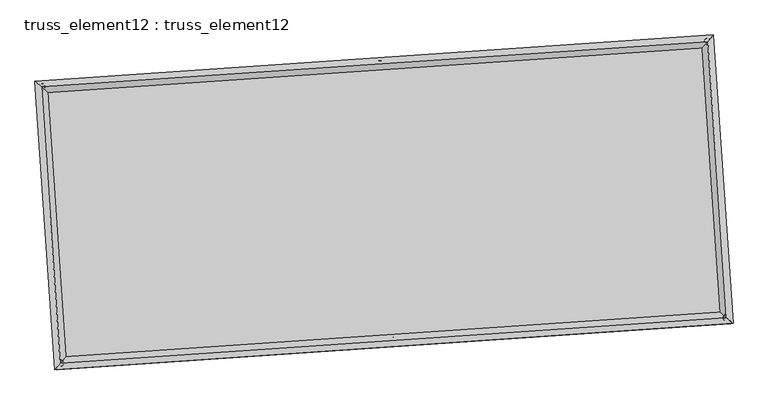
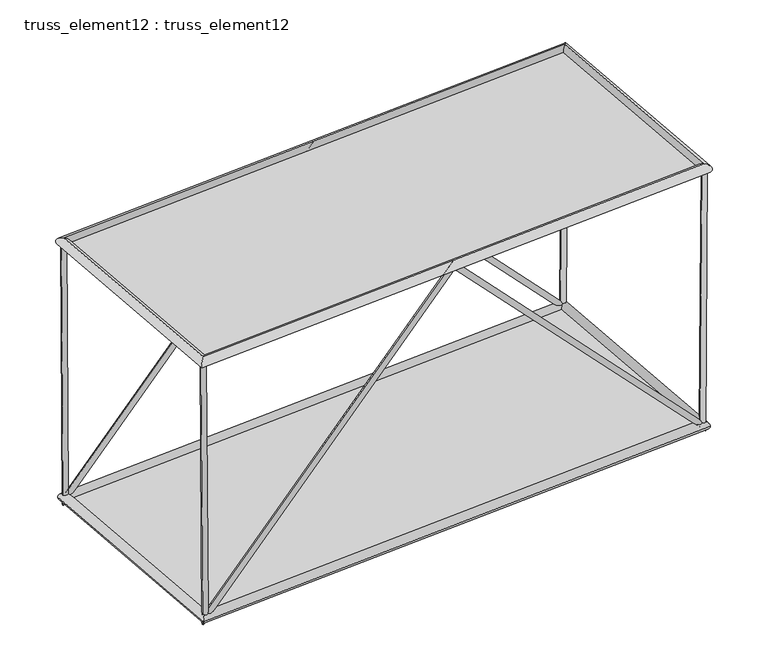
"""IFC4 building model written with IfcOpenShell, lengths in millimetres: plate geometry, truss_element12 : truss_element12."""

import ifcopenshell
import ifcopenshell.guid

model = None  # the IFC model being written
_history = None  # IfcOwnerHistory: only IFC2X3 demands one
_inside = {}  # id of a spatial element -> (the spatial element, [elements in it])
_under = {}  # id of a project, library or spatial element -> (it, [spatial elements below it])
_declared = {}  # id of a project -> (the project, [libraries it declares])
_typed = {}  # id of a type object -> (the type object, [elements of that type])
_made_of = {}  # id of a material, layer set ... -> (it, [elements and type objects made of it])


def new_model(schema):
    """Start an empty IFC model of exactly this schema.

    Asked for "IFC4X3", IfcOpenShell would pick the latest addendum, in which some entities
    have other attributes; the version numbers below select the first issue.
    IFC2X3 requires an IfcOwnerHistory on every rooted entity: one is made here for all.
    """
    global model, _history
    if schema == "IFC4X3":
        model = ifcopenshell.file(schema_version=(4, 3, 0, 0))
    else:
        model = ifcopenshell.file(schema=schema)
    _inside.clear()
    _under.clear()
    _declared.clear()
    _typed.clear()
    _made_of.clear()
    _history = None
    if model.schema == "IFC2X3":
        org = make("IfcOrganization", Name="unknown")
        user = make(
            "IfcPersonAndOrganization",
            ThePerson=make("IfcPerson", FamilyName="unknown"),
            TheOrganization=org,
        )
        app = make(
            "IfcApplication",
            ApplicationDeveloper=org,
            Version="unknown",
            ApplicationFullName="unknown",
            ApplicationIdentifier="unknown",
        )
        _history = make(
            "IfcOwnerHistory",
            OwningUser=user,
            OwningApplication=app,
            ChangeAction="ADDED",
            CreationDate=0,
        )
    return model


def make(cls, **values):
    """One entity of the class cls with the attributes given. An attribute that is None is left unset."""
    return model.create_entity(
        cls, **{name: value for name, value in values.items() if value is not None}
    )


def rooted(cls, **values):
    """An entity with a GlobalId (a new one), such as an element, a storey or a relation."""
    return make(cls, GlobalId=ifcopenshell.guid.new(), OwnerHistory=_history, **values)


def si_unit(unit_type, name, prefix=None):
    """IfcSIUnit, for example si_unit("LENGTHUNIT", "METRE", prefix="MILLI")."""
    return make("IfcSIUnit", UnitType=unit_type, Prefix=prefix, Name=name)


def assignment(units):
    """IfcUnitAssignment: the units of a project."""
    return None if units is None else make("IfcUnitAssignment", Units=units)


def point(xyz):
    """IfcCartesianPoint."""
    return None if xyz is None else make("IfcCartesianPoint", Coordinates=xyz)


def direction(xyz):
    """IfcDirection."""
    return None if xyz is None else make("IfcDirection", DirectionRatios=xyz)


def frame(location, z_axis=None, x_axis=None):
    """IfcAxis2Placement3D, a coordinate frame: its origin and axes. An axis left out is left unset."""
    return make(
        "IfcAxis2Placement3D",
        Location=point(location),
        Axis=direction(z_axis),
        RefDirection=direction(x_axis),
    )


def origin():
    """The frame at (0, 0, 0) with its axes left unset."""
    return frame((0.0, 0.0, 0.0))


def origin_with_axes():
    """The frame at (0, 0, 0) with the z axis (0, 0, 1) and the x axis (1, 0, 0) written out."""
    return frame((0.0, 0.0, 0.0), z_axis=(0.0, 0.0, 1.0), x_axis=(1.0, 0.0, 0.0))


def place(relative_to, where):
    """IfcLocalPlacement: puts the frame where relative to a parent placement (None: the world)."""
    return make(
        "IfcLocalPlacement", PlacementRelTo=relative_to, RelativePlacement=where
    )


def context(
    kind, dimensions, precision=None, world=None, true_north=None, identifier=None
):
    """IfcGeometricRepresentationContext, for example the 3D "Model" context."""
    return make(
        "IfcGeometricRepresentationContext",
        ContextIdentifier=identifier,
        ContextType=kind,
        CoordinateSpaceDimension=dimensions,
        Precision=precision,
        WorldCoordinateSystem=world,
        TrueNorth=true_north,
    )


def project(units=None, contexts=None):
    """IfcProject with its units and contexts."""
    return rooted(
        "IfcProject",
        Name="project",
        RepresentationContexts=contexts,
        UnitsInContext=assignment(units),
    )


def spatial(cls, under=None, at=None, **own):
    """A site, building, storey or space (cls), placed at a placement, below another one or the project."""
    s = rooted(cls, ObjectPlacement=at, **own)
    if under is not None:
        _under.setdefault(under.id(), (under, []))[1].append(s)
    return s


def polyline(points):
    """IfcPolyline through the points."""
    return make("IfcPolyline", Points=[point(p) for p in points])


def circle_curve(where, radius):
    """IfcCircle in the frame where."""
    return make("IfcCircle", Position=where, Radius=radius)


def ellipse_curve(where, semi_axis1, semi_axis2):
    """IfcEllipse in the frame where."""
    return make(
        "IfcEllipse", Position=where, SemiAxis1=semi_axis1, SemiAxis2=semi_axis2
    )


def outline(outer, holes=None, kind="AREA"):
    """IfcArbitraryClosedProfileDef: a profile drawn as a closed curve; with holes, ...WithVoids."""
    if holes is None:
        return make("IfcArbitraryClosedProfileDef", ProfileType=kind, OuterCurve=outer)
    return make(
        "IfcArbitraryProfileDefWithVoids",
        ProfileType=kind,
        OuterCurve=outer,
        InnerCurves=holes,
    )


def extrude(swept, where, along, depth):
    """IfcExtrudedAreaSolid: the profile swept, set in the frame where, extruded along a direction by depth."""
    return make(
        "IfcExtrudedAreaSolid",
        SweptArea=swept,
        Position=where,
        ExtrudedDirection=direction(along),
        Depth=depth,
    )


def shape(context_of_items, identifier, shape_type, items):
    """IfcShapeRepresentation: the items that make up one representation, for example the "Body"."""
    return make(
        "IfcShapeRepresentation",
        ContextOfItems=context_of_items,
        RepresentationIdentifier=identifier,
        RepresentationType=shape_type,
        Items=items,
    )


def source(mapping_origin, context_of_items, identifier, shape_type, items):
    """IfcRepresentationMap: a shape defined once, which mapped items show again and again."""
    return make(
        "IfcRepresentationMap",
        MappingOrigin=mapping_origin,
        MappedRepresentation=shape(context_of_items, identifier, shape_type, items),
    )


def transform(
    local_origin,
    x_axis=None,
    y_axis=None,
    z_axis=None,
    scale=None,
    scale2=None,
    scale3=None,
    uniform=True,
):
    """IfcCartesianTransformationOperator3D, or its non-uniform kind. x_axis, y_axis, z_axis: its Axis1, 2, 3."""
    if uniform:
        return make(
            "IfcCartesianTransformationOperator3D",
            Axis1=direction(x_axis),
            Axis2=direction(y_axis),
            LocalOrigin=point(local_origin),
            Scale=scale,
            Axis3=direction(z_axis),
        )
    return make(
        "IfcCartesianTransformationOperator3DnonUniform",
        Axis1=direction(x_axis),
        Axis2=direction(y_axis),
        LocalOrigin=point(local_origin),
        Scale=scale,
        Axis3=direction(z_axis),
        Scale2=scale2,
        Scale3=scale3,
    )


def mapped(mapping_source, mapping_target):
    """IfcMappedItem: shows the shape of a source again, moved by a transform."""
    return make(
        "IfcMappedItem", MappingSource=mapping_source, MappingTarget=mapping_target
    )


def made_of(thing, what):
    """Note that an element or type object is made of a material, layer set ...; save() writes the relation."""
    if what is not None:
        _made_of.setdefault(what.id(), (what, []))[1].append(thing)
    return thing


def element(
    cls,
    number,
    at=None,
    inside=None,
    cuts=None,
    type_object=None,
    material=None,
    context=None,
    identifier="Body",
    shape_type=None,
    held_by="IfcProductDefinitionShape",
    body=None,
    shapes=None,
    **own,
):
    """One element of the class cls, such as IfcWall. Its Tag is "e" and its number.

    at: its placement. inside: the storey or other place that contains it. cuts: it is an
    opening in that element (IfcRelVoidsElement). A single representation is given by context,
    identifier, shape_type and body (its items); several are given by shapes. held_by: the class
    of the entity that holds the representations. save() writes the other relations.
    """
    e = rooted(cls, Tag="e%d" % number, ObjectPlacement=at, **own)
    if body is not None:
        shapes = [shape(context, identifier, shape_type, body)]
    if shapes is not None:
        e.Representation = make(held_by, Representations=shapes)
    if inside is not None:
        _inside.setdefault(inside.id(), (inside, []))[1].append(e)
    if cuts is not None:
        rooted(
            "IfcRelVoidsElement", RelatingBuildingElement=cuts, RelatedOpeningElement=e
        )
    if type_object is not None:
        _typed.setdefault(type_object.id(), (type_object, []))[1].append(e)
    return made_of(e, material)


def aggregate(whole, parts):
    """IfcRelAggregates: a whole, such as a stair, and the parts it consists of."""
    return rooted("IfcRelAggregates", RelatingObject=whole, RelatedObjects=parts)


def save(model, path):
    """Write the relations noted so far, then the file.

    IfcRelAggregates (storeys below a building ...), IfcRelContainedInSpatialStructure (elements
    in a storey), IfcRelDefinesByType, IfcRelAssociatesMaterial and IfcRelDeclares: one each for
    every whole, place, type object, material and project.
    """
    for whole, parts in _under.values():
        aggregate(whole, parts)
    for where, things in _inside.values():
        rooted(
            "IfcRelContainedInSpatialStructure",
            RelatedElements=things,
            RelatingStructure=where,
        )
    for kind, things in _typed.values():
        rooted("IfcRelDefinesByType", RelatedObjects=things, RelatingType=kind)
    for what, things in _made_of.values():
        rooted("IfcRelAssociatesMaterial", RelatedObjects=things, RelatingMaterial=what)
    for by, libraries in _declared.values():
        rooted("IfcRelDeclares", RelatingContext=by, RelatedDefinitions=libraries)
    model.write(path)


def plane_surface(at):
    """IfcPlane: the flat surface through the origin of the frame at, square to its z axis."""
    return make("IfcPlane", Position=at)


def cylinder_surface(at, radius):
    """IfcCylindricalSurface: all points at the distance radius from the z axis of the frame at."""
    return make("IfcCylindricalSurface", Position=at, Radius=radius)


def advanced_brep(points, edges, surfaces, faces):
    """IfcAdvancedBrep: a solid bounded by faces that lie on surfaces and meet in shared edges.

    An edge is (start, end): straight between two places in points (the first is 0);
    or (start, end, curve); or (start, end, curve, False) where it runs against its curve.
    A face is (place in surfaces, loops), or (place, loops, False) where it looks against
    its surface's normal. A loop lists edges by number (the first is 1), with a minus sign
    where the edge is run from its end to its start. The first loop is the outer one.
    """
    corners = [point(p) for p in points]
    vertices = [make("IfcVertexPoint", VertexGeometry=c) for c in corners]
    made = []
    for start, end, *more in edges:
        made.append(
            make(
                "IfcEdgeCurve",
                EdgeStart=vertices[start],
                EdgeEnd=vertices[end],
                EdgeGeometry=more[0] if more else make("IfcPolyline", Points=[corners[start], corners[end]]),
                SameSense=more[1] if len(more) > 1 else True,
            )
        )
    hull = []
    for where, loops, *sense in faces:
        bounds = []
        for j, loop in enumerate(loops):
            ring = [make("IfcOrientedEdge", EdgeElement=made[abs(k) - 1], Orientation=k > 0) for k in loop]
            bounds.append(
                make(
                    "IfcFaceOuterBound" if j == 0 else "IfcFaceBound",
                    Bound=make("IfcEdgeLoop", EdgeList=ring),
                    Orientation=True,
                )
            )
        hull.append(make("IfcAdvancedFace", Bounds=bounds, FaceSurface=surfaces[where], SameSense=sense[0] if sense else True))
    return make("IfcAdvancedBrep", Outer=make("IfcClosedShell", CfsFaces=hull))


def truss_element12_truss_element12_8e9da1f8(model_context):
    return source(origin(), model_context, "Body", "SolidModel", [
        advanced_brep(
        [(-3698.7518615, 2273.9185866, 5000.223301), (-3797.8529392, 2260.5574847, 4999.5470243), (-3665.7745625, 2276.1671833, 123.3293266), (-3763.2123204, 2262.9194968, -123.3293266), (1063.9844604, 2598.6714715, 5072.0064402), (1064.4287053, 2592.0979868, 4927.7602832), (5793.2263236, 2921.1404966, 123.3255902), (5891.5346534, 2921.2399919, -123.3255902), (5826.7168605, 2923.424089, 5000.224961), (5926.7142716, 2923.6387563, 4999.5381605)],
        [
            (0, 1, circle_curve(frame((-3748.3024003, 2267.2380357, 4999.8851627), z_axis=(-0.0067617917796413095, -0.00046106087747684727, 0.9999770325336459), x_axis=(-0.13361106793445865, 0.9910337446995272, -0.0004465335886331621)), 50.0)),
            (1, 0, circle_curve(frame((-3748.3024003, 2267.2380357, 4999.8851627), z_axis=(-0.0067617917796413095, -0.00046106087747684727, 0.9999770325336459), x_axis=(-0.13361106793445865, 0.9910337446995272, -0.0004465335886331621)), 50.0)),
            (0, 2),
            (2, 3, ellipse_curve(frame((-3714.4934414, 2269.54334, 0.0), z_axis=(-0.9270371329382548, -0.06321113809700207, 0.3696031739231987), x_axis=(0.3687469497597502, 0.025143452765731104, 0.9291896974385251)), 133.0168379, 50.0)),
            (3, 1),
            (3, 2, ellipse_curve(frame((-3714.4934414, 2269.54334, 0.0), z_axis=(-0.9270371329382548, -0.06321113809700207, 0.3696031739231987), x_axis=(0.3687469497597502, 0.025143452765731104, 0.9291896974385251)), 133.0168379, 50.0)),
            (2, 4),
            (4, 5, ellipse_curve(frame((1064.2065829, 2595.3847292, 4999.8833617), z_axis=(-0.9976833956976204, -0.06802823820297674, 2.7500260085138387e-05), x_axis=(-2.74365528747556e-05, -1.8707942443931063e-06, -0.9999999996218679)), 72.2801261, 50.0)),
            (5, 3),
            (5, 4, ellipse_curve(frame((1064.2065829, 2595.3847292, 4999.8833617), z_axis=(-0.9976833956976204, -0.06802823820297674, 2.7500260085138387e-05), x_axis=(-2.74365528747556e-05, -1.8707942443931063e-06, -0.9999999996218679)), 72.2801261, 50.0)),
            (4, 6),
            (6, 7, ellipse_curve(frame((5842.3804885, 2921.1902443, 0.0), z_axis=(-0.9270667165570741, -0.0632131552915117, -0.3695286187160294), x_axis=(-0.3686725672674666, -0.0251383809063366, 0.9292193497500056)), 133.0085635, 50.0)),
            (7, 5),
            (7, 6, ellipse_curve(frame((5842.3804885, 2921.1902443, 0.0), z_axis=(-0.9270667165570741, -0.0632131552915117, -0.3695286187160294), x_axis=(-0.3686725672674666, -0.0251383809063366, 0.9292193497500056)), 133.0085635, 50.0)),
            (8, 9, circle_curve(frame((5876.715566, 2923.5314227, 4999.8815607), z_axis=(0.0068670155092968675, 0.0004682356836093084, 0.9999763121461127), x_axis=(-0.00214983747870396, 0.9999975862733836, -0.0004534823281307776)), 50.0)),
            (9, 8, circle_curve(frame((5876.715566, 2923.5314227, 4999.8815607), z_axis=(0.0068670155092968675, 0.0004682356836093084, 0.9999763121461127), x_axis=(-0.00214983747870396, 0.9999975862733836, -0.0004534823281307776)), 50.0)),
            (6, 8),
            (9, 7),
        ],
        [
            plane_surface(frame((-3748.3024003, 2317.2380303, 4999.9082162), z_axis=(-0.006761791779640632, -0.0004610608774721699, 0.9999770325336457), x_axis=(0.9999771388246477, -3.1176689248013658e-06, 0.006761791060906577))),
            cylinder_surface(frame((-3748.3024003, 2267.2380357, 4999.8851627), z_axis=(-0.006761791779641308, -0.00046106087747684716, 0.9999770325336457), x_axis=(-0.13361106793445865, 0.9910337446995272, -0.0004465335886331621)), 50.0),
            cylinder_surface(frame((-3714.4934414, 2269.54334, 0.0), z_axis=(-0.6901703766804573, -0.0470600944026198, -0.7221150868577476), x_axis=(-0.020414252830953418, 0.9987522052200565, -0.045577306298510874)), 50.0),
            cylinder_surface(frame((1064.2065829, 2595.3847292, 4999.8833617), z_axis=(-0.6901307509390454, -0.04705739247394453, 0.7221531336370857), x_axis=(-0.11534910612614199, 0.9922789584550205, -0.045574689503274965)), 50.0),
            plane_surface(frame((5876.715566, 2873.5314282, 4999.9049731), z_axis=(0.006867015509297537, 0.00046823568361033024, 0.9999763121461126), x_axis=(0.9999764217710311, -3.215457516247967e-06, -0.006867014756483772))),
            cylinder_surface(frame((5842.3804885, 2921.1902443, 0.0), z_axis=(-0.0068670155092968675, -0.0004682356836093084, -0.9999763121461127), x_axis=(-0.00214983747870396, 0.9999975862733836, -0.0004534823281307776)), 50.0),
        ],
        [
            (0, [[1, 2]]),
            (1, [[-1, 3, 4, 5]]),
            (1, [[-2, -5, 6, -3]]),
            (2, [[-4, 7, 8, 9]]),
            (2, [[-6, -9, 10, -7]]),
            (3, [[-8, 11, 12, 13]]),
            (3, [[-10, -13, 14, -11]]),
            (4, [[15, 16]]),
            (5, [[-12, 17, -16, 18]]),
            (5, [[-14, -18, -15, -17]]),
        ],
    ),
        advanced_brep(
        [(-3426.6389085, -1716.8149977, 5000.223301), (-3525.7399863, -1730.1760996, 4999.5470243), (-3393.6616095, -1714.566401, 123.3293266), (-3491.0993675, -1727.8140875, -123.3293266), (1336.0974133, -1392.0621128, 5072.0064402), (1336.5416582, -1398.6355975, 4927.7602832), (6065.3392765, -1069.5930877, 123.3255902), (6163.6476063, -1069.4935924, -123.3255902), (6098.8298134, -1067.3094953, 5000.224961), (6198.8272245, -1067.094828, 4999.5381605)],
        [
            (0, 1, circle_curve(frame((-3476.1894474, -1723.4955486, 4999.8851627), z_axis=(-0.006761791779640981, -0.00046106087747676796, 0.9999770325336458), x_axis=(-0.13361106793445865, 0.9910337446995272, -0.0004465335886331968)), 50.0)),
            (1, 0, circle_curve(frame((-3476.1894474, -1723.4955486, 4999.8851627), z_axis=(-0.006761791779640981, -0.00046106087747676796, 0.9999770325336458), x_axis=(-0.13361106793445865, 0.9910337446995272, -0.0004465335886331968)), 50.0)),
            (0, 2),
            (2, 3, ellipse_curve(frame((-3442.3804885, -1721.1902443, 0.0), z_axis=(-0.9270371329382548, -0.06321113809700199, 0.3696031739231986), x_axis=(0.3687469497597501, 0.025143452765731125, 0.9291896974385251)), 133.0168379, 50.0)),
            (3, 1),
            (3, 2, ellipse_curve(frame((-3442.3804885, -1721.1902443, 0.0), z_axis=(-0.9270371329382548, -0.06321113809700199, 0.3696031739231986), x_axis=(0.3687469497597501, 0.025143452765731125, 0.9291896974385251)), 133.0168379, 50.0)),
            (2, 4),
            (4, 5, ellipse_curve(frame((1336.3195358, -1395.3488551, 4999.8833617), z_axis=(-0.9976833956976204, -0.0680282382029767, 2.7500260084977895e-05), x_axis=(-2.7436552874601853e-05, -1.8707942444027149e-06, -0.9999999996218678)), 72.2801261, 50.0)),
            (5, 3),
            (5, 4, ellipse_curve(frame((1336.3195358, -1395.3488551, 4999.8833617), z_axis=(-0.9976833956976204, -0.0680282382029767, 2.7500260084977895e-05), x_axis=(-2.7436552874601853e-05, -1.8707942444027149e-06, -0.9999999996218678)), 72.2801261, 50.0)),
            (4, 6),
            (6, 7, ellipse_curve(frame((6114.4934414, -1069.54334, 0.0), z_axis=(-0.9270667165570744, -0.06321315529151138, -0.3695286187160292), x_axis=(-0.36867256726746617, -0.025138380906336657, 0.9292193497500058)), 133.0085635, 50.0)),
            (7, 5),
            (7, 6, ellipse_curve(frame((6114.4934414, -1069.54334, 0.0), z_axis=(-0.9270667165570744, -0.06321315529151138, -0.3695286187160292), x_axis=(-0.36867256726746617, -0.025138380906336657, 0.9292193497500058)), 133.0085635, 50.0)),
            (8, 9, circle_curve(frame((6148.828519, -1067.2021616, 4999.8815607), z_axis=(0.0068670155092972595, 0.00046823568360912634, 0.9999763121461127), x_axis=(-0.0021498374787036058, 0.9999975862733835, -0.0004534823281305971)), 50.0)),
            (9, 8, circle_curve(frame((6148.828519, -1067.2021616, 4999.8815607), z_axis=(0.0068670155092972595, 0.00046823568360912634, 0.9999763121461127), x_axis=(-0.0021498374787036058, 0.9999975862733835, -0.0004534823281305971)), 50.0)),
            (6, 8),
            (9, 7),
        ],
        [
            plane_surface(frame((-3476.1894474, -1673.495554, 4999.9082162), z_axis=(-0.006761791779640632, -0.00046106087747216866, 0.9999770325336457), x_axis=(0.9999771388246477, -3.1176689248013658e-06, 0.006761791060906577))),
            cylinder_surface(frame((-3476.1894474, -1723.4955486, 4999.8851627), z_axis=(-0.006761791779640981, -0.00046106087747676796, 0.9999770325336458), x_axis=(-0.13361106793445865, 0.9910337446995272, -0.0004465335886331968)), 50.0),
            cylinder_surface(frame((-3442.3804885, -1721.1902443, 0.0), z_axis=(-0.6901703766804571, -0.047060094402619775, -0.7221150868577478), x_axis=(-0.020414252830953338, 0.9987522052200565, -0.04557730629851091)), 50.0),
            cylinder_surface(frame((1336.3195358, -1395.3488551, 4999.8833617), z_axis=(-0.6901307509390455, -0.04705739247394449, 0.7221531336370857), x_axis=(-0.11534910612614203, 0.9922789584550205, -0.04557468950327508)), 50.0),
            plane_surface(frame((6148.828519, -1117.2021561, 4999.9049731), z_axis=(0.006867015509297537, 0.0004682356836103296, 0.9999763121461126), x_axis=(0.9999764217710311, -3.215457516247967e-06, -0.006867014756483772))),
            cylinder_surface(frame((6114.4934414, -1069.54334, 0.0), z_axis=(-0.0068670155092972595, -0.00046823568360912634, -0.9999763121461127), x_axis=(-0.0021498374787036058, 0.9999975862733835, -0.0004534823281305971)), 50.0),
        ],
        [
            (0, [[1, 2]]),
            (1, [[-1, 3, 4, 5]]),
            (1, [[-2, -5, 6, -3]]),
            (2, [[-4, 7, 8, 9]]),
            (2, [[-6, -9, 10, -7]]),
            (3, [[-8, 11, 12, 13]]),
            (3, [[-10, -13, 14, -11]]),
            (4, [[15, 16]]),
            (5, [[-12, 17, -16, 18]]),
            (5, [[-14, -18, -15, -17]]),
        ],
    ),
        advanced_brep(
        [(-3476.1903983, -1723.4966025, 4909.8851627), (-3476.1884965, -1723.4944948, 5089.8851627), (-3748.3013152, 2267.2371206, 5089.8851627), (-3748.3034854, 2267.2389507, 4909.8851627), (5876.7146822, 2923.5303734, 5089.8815607), (5876.7164499, 2923.532472, 4909.8815607), (6148.8275009, -1067.201242, 5089.8815607), (6148.829537, -1067.2030813, 4909.8815607)],
        [
            (0, 1, ellipse_curve(frame((-3476.1894474, -1723.4955486, 4999.8851627), z_axis=(-0.753571923405407, 0.657365466278086, 2.6400514504974096e-07), x_axis=(-0.6573654662780334, -0.7535719234054531, 2.640051450497678e-07)), 127.2792206, 90.0)),
            (1, 2),
            (2, 3, ellipse_curve(frame((-3748.3024003, 2267.2380357, 4999.8851627), z_axis=(-0.6573654662780334, -0.7535719234054531, 2.640051450497922e-07), x_axis=(0.7535719234054074, -0.657365466278086, -2.6400514504976537e-07)), 127.2792206, 90.0)),
            (3, 0),
            (1, 0, ellipse_curve(frame((-3476.1894474, -1723.4955486, 4999.8851627), z_axis=(-0.753571923405407, 0.657365466278086, 2.6400514504974096e-07), x_axis=(-0.6573654662780334, -0.7535719234054531, 2.640051450497678e-07)), 127.2792206, 90.0)),
            (3, 2, ellipse_curve(frame((-3748.3024003, 2267.2380357, 4999.8851627), z_axis=(-0.6573654662780334, -0.7535719234054531, 2.640051450497922e-07), x_axis=(0.7535719234054074, -0.657365466278086, -2.6400514504976537e-07)), 127.2792206, 90.0)),
            (2, 4),
            (4, 5, ellipse_curve(frame((5876.715566, 2923.5314227, 4999.8815607), z_axis=(-0.7535719234054071, 0.6573654662780859, 2.6400514504978967e-07), x_axis=(-0.6573654662780337, -0.7535719234054528, 2.64005145049768e-07)), 127.2792206, 90.0)),
            (5, 3),
            (5, 4, ellipse_curve(frame((5876.715566, 2923.5314227, 4999.8815607), z_axis=(-0.7535719234054071, 0.6573654662780859, 2.6400514504978967e-07), x_axis=(-0.6573654662780337, -0.7535719234054528, 2.64005145049768e-07)), 127.2792206, 90.0)),
            (4, 6),
            (6, 7, ellipse_curve(frame((6148.828519, -1067.2021616, 4999.8815607), z_axis=(0.6573654662780337, 0.7535719234054529, -2.640051450497436e-07), x_axis=(-0.753571923405407, 0.6573654662780861, 2.640051450497652e-07)), 127.2792206, 90.0)),
            (7, 5),
            (7, 6, ellipse_curve(frame((6148.828519, -1067.2021616, 4999.8815607), z_axis=(0.6573654662780337, 0.7535719234054529, -2.640051450497436e-07), x_axis=(-0.753571923405407, 0.6573654662780861, 2.640051450497652e-07)), 127.2792206, 90.0)),
            (6, 1),
            (0, 7),
        ],
        [
            cylinder_surface(frame((-3476.1894474, -1723.4955486, 4999.8851627), z_axis=(0.06802823822870037, -0.9976833960748768, 0.0), x_axis=(-0.997683396010759, -0.06802823822432842, 1.1337253567217425e-05)), 90.0),
            cylinder_surface(frame((-3748.3024003, 2267.2380357, 4999.8851627), z_axis=(-0.9976833960748074, -0.06802823822869285, 3.733596566656734e-07), x_axis=(-0.06802823822052487, 0.9976833960151911, 1.0963893910574207e-05)), 90.0),
            cylinder_surface(frame((5876.715566, 2923.5314227, 4999.8815607), z_axis=(-0.06802823822870019, 0.9976833960748768, 0.0), x_axis=(0.997683396018927, 0.06802823822488518, 1.0590534253930997e-05)), 90.0),
            cylinder_surface(frame((6148.828519, -1067.2021616, 4999.8815607), z_axis=(0.9976833960748073, 0.06802823822869236, -3.733596566656388e-07), x_axis=(0.06802823822869236, -0.9976833960146341, 1.0963893910574209e-05)), 90.0),
        ],
        [
            (0, [[1, 2, 3, 4]]),
            (0, [[5, -4, 6, -2]]),
            (1, [[-3, 7, 8, 9]]),
            (1, [[-6, -9, 10, -7]]),
            (2, [[-8, 11, 12, 13]]),
            (2, [[-10, -13, 14, -11]]),
            (3, [[-12, 15, -1, 16]]),
            (3, [[-14, -16, -5, -15]]),
        ],
    ),
        advanced_brep(
        [(-3358.7115243, -1625.2761972, 0.0), (-3526.0494527, -1817.1042913, 0.0), (-3810.4074885, 2353.2123043, 0.0), (-3618.5793943, 2185.8743758, 0.0), (5926.0494527, 3017.1042913, 0.0), (5758.7115243, 2825.2761972, 0.0), (6210.4074885, -1153.2123043, 0.0), (6018.5793943, -985.8743758, 0.0)],
        [
            (0, 1, ellipse_curve(frame((-3442.3804885, -1721.1902443, 0.0), z_axis=(-0.7535719234054583, 0.6573654662780805, 0.0), x_axis=(-0.6573654662780805, -0.7535719234054583, 0.0)), 127.2792206, 90.0)),
            (1, 2),
            (2, 3, ellipse_curve(frame((-3714.4934414, 2269.54334, 0.0), z_axis=(-0.6573654662780805, -0.7535719234054583, 0.0), x_axis=(0.7535719234054583, -0.6573654662780805, 0.0)), 127.2792206, 90.0)),
            (3, 0),
            (1, 0, ellipse_curve(frame((-3442.3804885, -1721.1902443, 0.0), z_axis=(-0.7535719234054583, 0.6573654662780805, 0.0), x_axis=(-0.6573654662780805, -0.7535719234054583, 0.0)), 127.2792206, 90.0)),
            (3, 2, ellipse_curve(frame((-3714.4934414, 2269.54334, 0.0), z_axis=(-0.6573654662780805, -0.7535719234054583, 0.0), x_axis=(0.7535719234054583, -0.6573654662780805, 0.0)), 127.2792206, 90.0)),
            (2, 4),
            (4, 5, ellipse_curve(frame((5842.3804885, 2921.1902443, 0.0), z_axis=(-0.7535719234054583, 0.6573654662780805, 0.0), x_axis=(-0.6573654662780805, -0.7535719234054583, 0.0)), 127.2792206, 90.0)),
            (5, 3),
            (5, 4, ellipse_curve(frame((5842.3804885, 2921.1902443, 0.0), z_axis=(-0.7535719234054583, 0.6573654662780805, 0.0), x_axis=(-0.6573654662780805, -0.7535719234054583, 0.0)), 127.2792206, 90.0)),
            (4, 6),
            (6, 7, ellipse_curve(frame((6114.4934414, -1069.54334, 0.0), z_axis=(0.6573654662780806, 0.7535719234054583, 0.0), x_axis=(-0.7535719234054584, 0.6573654662780802, 0.0)), 127.2792206, 90.0)),
            (7, 5),
            (7, 6, ellipse_curve(frame((6114.4934414, -1069.54334, 0.0), z_axis=(0.6573654662780806, 0.7535719234054583, 0.0), x_axis=(-0.7535719234054584, 0.6573654662780802, 0.0)), 127.2792206, 90.0)),
            (6, 1),
            (0, 7),
        ],
        [
            cylinder_surface(frame((-3442.3804885, -1721.1902443, 0.0), z_axis=(0.06802823822870305, -0.9976833960748764, 0.0), x_axis=(-0.9976833960748764, -0.06802823822870305, 0.0)), 90.0),
            cylinder_surface(frame((-3714.4934414, 2269.54334, 0.0), z_axis=(-0.9976833960748767, -0.06802823822870038, 0.0), x_axis=(-0.06802823822870038, 0.9976833960748767, 0.0)), 90.0),
            cylinder_surface(frame((5842.3804885, 2921.1902443, 0.0), z_axis=(-0.06802823822870298, 0.9976833960748764, 0.0), x_axis=(0.9976833960748764, 0.06802823822870298, 0.0)), 90.0),
            cylinder_surface(frame((6114.4934414, -1069.54334, 0.0), z_axis=(0.9976833960748767, 0.06802823822870031, 0.0), x_axis=(0.06802823822870031, -0.9976833960748767, 0.0)), 90.0),
        ],
        [
            (0, [[1, 2, 3, 4]]),
            (0, [[5, -4, 6, -2]]),
            (1, [[-3, 7, 8, 9]]),
            (1, [[-6, -9, 10, -7]]),
            (2, [[-8, 11, 12, 13]]),
            (2, [[-10, -13, 14, -11]]),
            (3, [[-12, 15, -1, 16]]),
            (3, [[-14, -16, -5, -15]]),
        ],
    ),
        extrude(outline(polyline([(-3442.3804885, -1721.1902443), (-3714.4934414, 2269.54334), (5842.3804885, 2921.1902443), (6114.4934414, -1069.54334), (-3442.3804885, -1721.1902443)])), origin_with_axes(), (0.0, 0.0, 1.0), 20.0),
        extrude(outline(polyline([(-1999.9999999, 4823.6835474), (2000.0000001, 4823.6835474), (2000.0, -4823.6835474), (-2000.0, -4823.6835475), (-1999.9999999, 4823.6835474)])), frame((1200.2630593, 600.017937, 4999.8833617), z_axis=(3.724947302195416e-07, 2.5398999668638065e-08, 0.9999999999999303), x_axis=(-0.06802823822870314, 0.9976833960748764, 0.0)), (0.0, 0.0, 1.0), 20.0),
    ])


if __name__ == "__main__":
    model = new_model("IFC4")
    model_context = context("Model", 3, world=origin())
    ifc_project = project(units=[si_unit("LENGTHUNIT", "METRE", prefix="MILLI")], contexts=[model_context])
    site = spatial("IfcSite", under=ifc_project)
    building = spatial("IfcBuilding", under=site)
    placement = place(None, origin())
    truss_element12_truss_element12_shape = truss_element12_truss_element12_8e9da1f8(model_context)
    element("IfcPlate", 1, ObjectType="truss_element12 : truss_element12", at=placement, inside=building, context=model_context, shape_type="MappedRepresentation", body=[
        mapped(truss_element12_truss_element12_shape, transform((0.0, 0.0, 0.0), x_axis=(1.0, 0.0, 0.0), y_axis=(0.0, 1.0, 0.0), z_axis=(0.0, 0.0, 1.0))),
    ])
    save(model, "model.ifc")

# Revit data of these elements
# Type "truss_element12 : truss_element12"
#   steellbar1 = 90 mm
#   steelbar2 = 50 mm
#   offset1 = 5000 mm
#   M = Default Roof
# Element 1 (IfcPlate, "truss_element12 : truss_element12")
#   Materials on its faces: "Default Roof"
# Materials
#   "Default Roof": class "Miscellaneous", colour RGB 0 127 0, transparency 0, Comments = "Rendering appearance not upgraded Rendering appearance not upgraded ", Cost = 0
